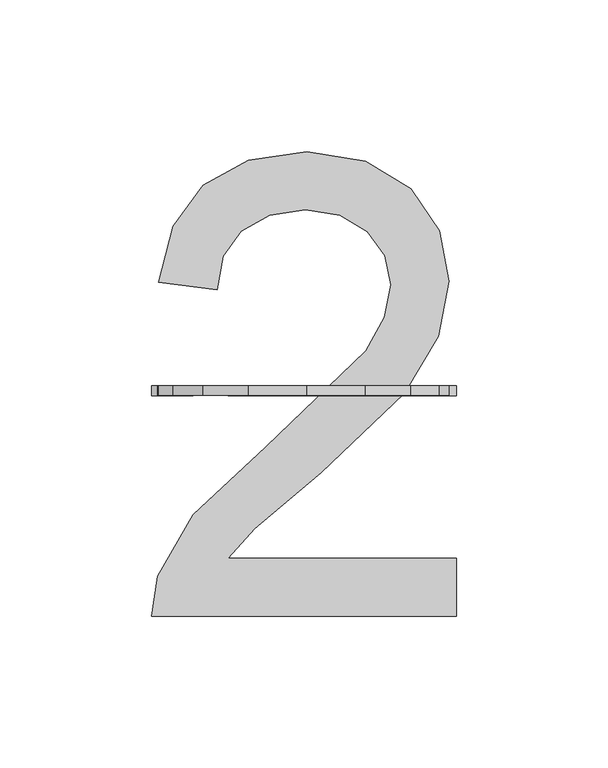
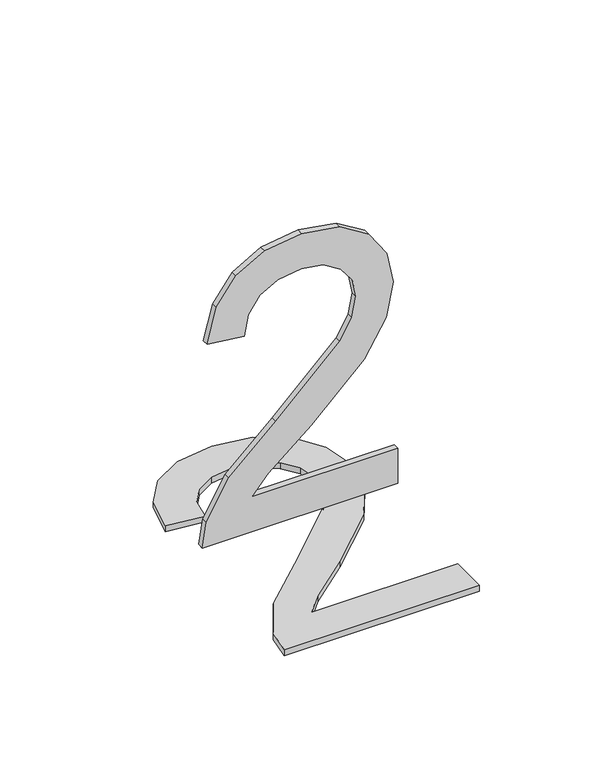
"""IFC4 building model written with IfcOpenShell, lengths in millimetres: proxy geometry, Grid Number1_FedEx : Grid Number1_FedEx."""

from ifc_helpers import new_model, si_unit, frame, origin, origin_with_axes, place, context, project, spatial, polyline, outline, extrude, source, transform, mapped, element, save


def entourage_08969285(model_context):
    return source(origin(), model_context, "Body", "SweptSolid", [
        extrude(outline(polyline([(-59.0355511, 165.720992), (-59.0355511, 146.5840649), (-159.5044183, 146.5840649), (-157.4486937, 159.7780791), (-145.8245056, 180.0923757), (-121.8659699, 202.2755129), (-88.8248692, 234.1579324), (-82.6296628, 245.1467148), (-80.5645941, 255.8364826), (-82.5128603, 265.4189625), (-88.3576591, 273.3848953), (-97.34211, 278.7531397), (-108.7093325, 280.5425545), (-120.6465514, 278.7951886), (-129.9206726, 273.5530909), (-135.9056344, 265.2274063), (-137.9753753, 254.2292798), (-157.1123024, 256.6213957), (-152.4729058, 275.1322612), (-142.4419042, 288.6533224), (-127.542573, 296.9229418), (-108.2981876, 299.6794816), (-88.9136391, 296.6145831), (-74.0423406, 287.4198877), (-64.5813354, 273.6839097), (-61.427667, 256.9951638), (-64.8289567, 238.8487222), (-76.135442, 220.0855632), (-103.5513326, 193.8657305), (-125.5662741, 175.4576512), (-134.2003174, 165.720992), (-59.0355511, 165.720992)])), origin_with_axes(), (0.0, 0.0, 1.0), 3.175),
        extrude(outline(polyline([(33.6168203, -59.0355511), (33.6168203, -134.2003174), (43.3534795, -125.5662741), (61.7615588, -103.5513326), (87.9813915, -76.135442), (106.7445505, -64.8289567), (124.8909921, -61.427667), (141.5797381, -64.5813354), (155.315716, -74.0423406), (164.5104114, -88.9136391), (167.5753099, -108.2981876), (164.8187701, -127.542573), (156.5491508, -142.4419042), (143.0280895, -152.4729058), (124.517224, -157.1123024), (122.1251081, -137.9753753), (133.1232346, -135.9056344), (141.4489192, -129.9206726), (146.6910169, -120.6465514), (148.4383828, -108.7093325), (146.648968, -97.34211), (141.2807236, -88.3576591), (133.3147908, -82.5128603), (123.7323109, -80.5645941), (113.0425431, -82.6296628), (102.0537607, -88.8248692), (70.1713412, -121.8659699), (47.988204, -145.8245056), (27.6739074, -157.4486937), (14.4798932, -159.5044183), (14.4798932, -59.0355511), (33.6168203, -59.0355511)])), frame((0.0, 219.3456765, 0.0), z_axis=(0.0, 1.0, 0.0), x_axis=(0.0, 0.0, 1.0)), (0.0, 0.0, 1.0), 3.175),
    ])


if __name__ == "__main__":
    model = new_model("IFC4")
    model_context = context("Model", 3, world=origin())
    ifc_project = project(units=[si_unit("LENGTHUNIT", "METRE", prefix="MILLI")], contexts=[model_context])
    site = spatial("IfcSite", under=ifc_project)
    building = spatial("IfcBuilding", under=site)
    placement = place(None, origin())
    entourage_shape = entourage_08969285(model_context)
    element("IfcBuildingElementProxy", 1, Name="Grid Number1_FedEx : Grid Number1_FedEx", ObjectType="Grid Number1_FedEx : Grid Number1_FedEx", at=placement, inside=building, context=model_context, shape_type="MappedRepresentation", body=[
        mapped(entourage_shape, transform((0.0, 0.0, 0.0), x_axis=(1.0, 0.0, 0.0), y_axis=(0.0, 1.0, 0.0), z_axis=(0.0, 0.0, 1.0))),
    ])
    save(model, "model.ifc")

# Revit data of these elements
# Type "Grid Number1_FedEx : Grid Number1_FedEx"
#   Grid [instance default] = "S.8"
#   Label Width [instance default] = 1' - 0"
#   Half Box Width2 [instance default] = 0' - 6.13846"
#   Half Box Width [instance default] = 0' - 6"
#   Robust [instance default] = yes
#   Height = 0
#   Assembly Code = ""
# Element 1 (IfcBuildingElementProxy, "Grid Number1_FedEx : Grid Number1_FedEx")
#   Grid = "2"
#   Robust = no
#   Materials on its faces: "Letter"
# Materials
#   "Letter": class "Unassigned", colour RGB 178 187 30, transparency 0, Comments = "Rendering appearance not upgraded "
